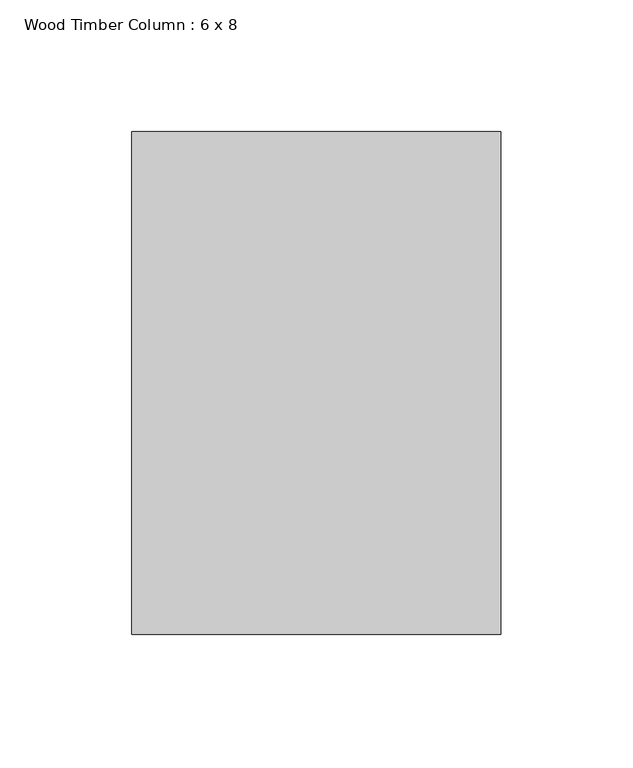
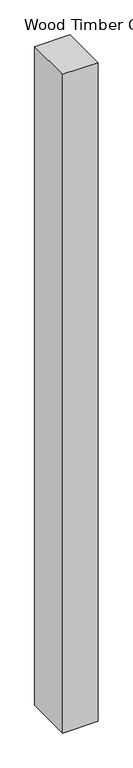
"""IFC4 building model written with IfcOpenShell, lengths in millimetres: column geometry, Wood Timber Column : 6 x 8."""

import ifcopenshell
import ifcopenshell.guid

model = None  # the IFC model being written
_history = None  # IfcOwnerHistory: only IFC2X3 demands one
_inside = {}  # id of a spatial element -> (the spatial element, [elements in it])
_under = {}  # id of a project, library or spatial element -> (it, [spatial elements below it])
_declared = {}  # id of a project -> (the project, [libraries it declares])
_typed = {}  # id of a type object -> (the type object, [elements of that type])
_made_of = {}  # id of a material, layer set ... -> (it, [elements and type objects made of it])


def new_model(schema):
    """Start an empty IFC model of exactly this schema.

    Asked for "IFC4X3", IfcOpenShell would pick the latest addendum, in which some entities
    have other attributes; the version numbers below select the first issue.
    IFC2X3 requires an IfcOwnerHistory on every rooted entity: one is made here for all.
    """
    global model, _history
    if schema == "IFC4X3":
        model = ifcopenshell.file(schema_version=(4, 3, 0, 0))
    else:
        model = ifcopenshell.file(schema=schema)
    _inside.clear()
    _under.clear()
    _declared.clear()
    _typed.clear()
    _made_of.clear()
    _history = None
    if model.schema == "IFC2X3":
        org = make("IfcOrganization", Name="unknown")
        user = make(
            "IfcPersonAndOrganization",
            ThePerson=make("IfcPerson", FamilyName="unknown"),
            TheOrganization=org,
        )
        app = make(
            "IfcApplication",
            ApplicationDeveloper=org,
            Version="unknown",
            ApplicationFullName="unknown",
            ApplicationIdentifier="unknown",
        )
        _history = make(
            "IfcOwnerHistory",
            OwningUser=user,
            OwningApplication=app,
            ChangeAction="ADDED",
            CreationDate=0,
        )
    return model


def make(cls, **values):
    """One entity of the class cls with the attributes given. An attribute that is None is left unset."""
    return model.create_entity(
        cls, **{name: value for name, value in values.items() if value is not None}
    )


def rooted(cls, **values):
    """An entity with a GlobalId (a new one), such as an element, a storey or a relation."""
    return make(cls, GlobalId=ifcopenshell.guid.new(), OwnerHistory=_history, **values)


def si_unit(unit_type, name, prefix=None):
    """IfcSIUnit, for example si_unit("LENGTHUNIT", "METRE", prefix="MILLI")."""
    return make("IfcSIUnit", UnitType=unit_type, Prefix=prefix, Name=name)


def assignment(units):
    """IfcUnitAssignment: the units of a project."""
    return None if units is None else make("IfcUnitAssignment", Units=units)


def point(xyz):
    """IfcCartesianPoint."""
    return None if xyz is None else make("IfcCartesianPoint", Coordinates=xyz)


def direction(xyz):
    """IfcDirection."""
    return None if xyz is None else make("IfcDirection", DirectionRatios=xyz)


def frame(location, z_axis=None, x_axis=None):
    """IfcAxis2Placement3D, a coordinate frame: its origin and axes. An axis left out is left unset."""
    return make(
        "IfcAxis2Placement3D",
        Location=point(location),
        Axis=direction(z_axis),
        RefDirection=direction(x_axis),
    )


def origin():
    """The frame at (0, 0, 0) with its axes left unset."""
    return frame((0.0, 0.0, 0.0))


def place(relative_to, where):
    """IfcLocalPlacement: puts the frame where relative to a parent placement (None: the world)."""
    return make(
        "IfcLocalPlacement", PlacementRelTo=relative_to, RelativePlacement=where
    )


def context(
    kind, dimensions, precision=None, world=None, true_north=None, identifier=None
):
    """IfcGeometricRepresentationContext, for example the 3D "Model" context."""
    return make(
        "IfcGeometricRepresentationContext",
        ContextIdentifier=identifier,
        ContextType=kind,
        CoordinateSpaceDimension=dimensions,
        Precision=precision,
        WorldCoordinateSystem=world,
        TrueNorth=true_north,
    )


def project(units=None, contexts=None):
    """IfcProject with its units and contexts."""
    return rooted(
        "IfcProject",
        Name="project",
        RepresentationContexts=contexts,
        UnitsInContext=assignment(units),
    )


def spatial(cls, under=None, at=None, **own):
    """A site, building, storey or space (cls), placed at a placement, below another one or the project."""
    s = rooted(cls, ObjectPlacement=at, **own)
    if under is not None:
        _under.setdefault(under.id(), (under, []))[1].append(s)
    return s


def polyline(points):
    """IfcPolyline through the points."""
    return make("IfcPolyline", Points=[point(p) for p in points])


def outline(outer, holes=None, kind="AREA"):
    """IfcArbitraryClosedProfileDef: a profile drawn as a closed curve; with holes, ...WithVoids."""
    if holes is None:
        return make("IfcArbitraryClosedProfileDef", ProfileType=kind, OuterCurve=outer)
    return make(
        "IfcArbitraryProfileDefWithVoids",
        ProfileType=kind,
        OuterCurve=outer,
        InnerCurves=holes,
    )


def extrude(swept, where, along, depth):
    """IfcExtrudedAreaSolid: the profile swept, set in the frame where, extruded along a direction by depth."""
    return make(
        "IfcExtrudedAreaSolid",
        SweptArea=swept,
        Position=where,
        ExtrudedDirection=direction(along),
        Depth=depth,
    )


def shape(context_of_items, identifier, shape_type, items):
    """IfcShapeRepresentation: the items that make up one representation, for example the "Body"."""
    return make(
        "IfcShapeRepresentation",
        ContextOfItems=context_of_items,
        RepresentationIdentifier=identifier,
        RepresentationType=shape_type,
        Items=items,
    )


def source(mapping_origin, context_of_items, identifier, shape_type, items):
    """IfcRepresentationMap: a shape defined once, which mapped items show again and again."""
    return make(
        "IfcRepresentationMap",
        MappingOrigin=mapping_origin,
        MappedRepresentation=shape(context_of_items, identifier, shape_type, items),
    )


def transform(
    local_origin,
    x_axis=None,
    y_axis=None,
    z_axis=None,
    scale=None,
    scale2=None,
    scale3=None,
    uniform=True,
):
    """IfcCartesianTransformationOperator3D, or its non-uniform kind. x_axis, y_axis, z_axis: its Axis1, 2, 3."""
    if uniform:
        return make(
            "IfcCartesianTransformationOperator3D",
            Axis1=direction(x_axis),
            Axis2=direction(y_axis),
            LocalOrigin=point(local_origin),
            Scale=scale,
            Axis3=direction(z_axis),
        )
    return make(
        "IfcCartesianTransformationOperator3DnonUniform",
        Axis1=direction(x_axis),
        Axis2=direction(y_axis),
        LocalOrigin=point(local_origin),
        Scale=scale,
        Axis3=direction(z_axis),
        Scale2=scale2,
        Scale3=scale3,
    )


def mapped(mapping_source, mapping_target):
    """IfcMappedItem: shows the shape of a source again, moved by a transform."""
    return make(
        "IfcMappedItem", MappingSource=mapping_source, MappingTarget=mapping_target
    )


def made_of(thing, what):
    """Note that an element or type object is made of a material, layer set ...; save() writes the relation."""
    if what is not None:
        _made_of.setdefault(what.id(), (what, []))[1].append(thing)
    return thing


def element(
    cls,
    number,
    at=None,
    inside=None,
    cuts=None,
    type_object=None,
    material=None,
    context=None,
    identifier="Body",
    shape_type=None,
    held_by="IfcProductDefinitionShape",
    body=None,
    shapes=None,
    **own,
):
    """One element of the class cls, such as IfcWall. Its Tag is "e" and its number.

    at: its placement. inside: the storey or other place that contains it. cuts: it is an
    opening in that element (IfcRelVoidsElement). A single representation is given by context,
    identifier, shape_type and body (its items); several are given by shapes. held_by: the class
    of the entity that holds the representations. save() writes the other relations.
    """
    e = rooted(cls, Tag="e%d" % number, ObjectPlacement=at, **own)
    if body is not None:
        shapes = [shape(context, identifier, shape_type, body)]
    if shapes is not None:
        e.Representation = make(held_by, Representations=shapes)
    if inside is not None:
        _inside.setdefault(inside.id(), (inside, []))[1].append(e)
    if cuts is not None:
        rooted(
            "IfcRelVoidsElement", RelatingBuildingElement=cuts, RelatedOpeningElement=e
        )
    if type_object is not None:
        _typed.setdefault(type_object.id(), (type_object, []))[1].append(e)
    return made_of(e, material)


def aggregate(whole, parts):
    """IfcRelAggregates: a whole, such as a stair, and the parts it consists of."""
    return rooted("IfcRelAggregates", RelatingObject=whole, RelatedObjects=parts)


def save(model, path):
    """Write the relations noted so far, then the file.

    IfcRelAggregates (storeys below a building ...), IfcRelContainedInSpatialStructure (elements
    in a storey), IfcRelDefinesByType, IfcRelAssociatesMaterial and IfcRelDeclares: one each for
    every whole, place, type object, material and project.
    """
    for whole, parts in _under.values():
        aggregate(whole, parts)
    for where, things in _inside.values():
        rooted(
            "IfcRelContainedInSpatialStructure",
            RelatedElements=things,
            RelatingStructure=where,
        )
    for kind, things in _typed.values():
        rooted("IfcRelDefinesByType", RelatedObjects=things, RelatingType=kind)
    for what, things in _made_of.values():
        rooted("IfcRelAssociatesMaterial", RelatedObjects=things, RelatingMaterial=what)
    for by, libraries in _declared.values():
        rooted("IfcRelDeclares", RelatingContext=by, RelatedDefinitions=libraries)
    model.write(path)


def wood_timber_column_6_x_8_dc19652e(model_context):
    return source(origin(), model_context, "Body", "SweptSolid", [
        extrude(outline(polyline([(69.85, -95.25), (-69.85, -95.25), (-69.85, 95.25), (69.85, 95.25), (69.85, -95.25)])), frame((0.0, 0.0, 2743.2), z_axis=(0.0, 0.0, 1.0), x_axis=(1.0, 0.0, 0.0)), (0.0, 0.0, 1.0), 2743.2),
    ])


if __name__ == "__main__":
    model = new_model("IFC4")
    model_context = context("Model", 3, world=origin())
    ifc_project = project(units=[si_unit("LENGTHUNIT", "METRE", prefix="MILLI")], contexts=[model_context])
    site = spatial("IfcSite", under=ifc_project)
    building = spatial("IfcBuilding", under=site)
    placement = place(None, origin())
    wood_timber_column_6_x_8_shape = wood_timber_column_6_x_8_dc19652e(model_context)
    element("IfcColumn", 1, ObjectType="Wood Timber Column : 6 x 8", at=placement, inside=building, context=model_context, shape_type="MappedRepresentation", body=[
        mapped(wood_timber_column_6_x_8_shape, transform((0.0, 0.0, 0.0), x_axis=(1.0, 0.0, 0.0), y_axis=(0.0, 1.0, 0.0), z_axis=(0.0, 0.0, 1.0))),
    ])
    save(model, "model.ifc")

# Revit data of these elements
# Type "Wood Timber Column : 6 x 8"
#   Assembly Code = "B1010200"
#   Depth = 0' - 7 1/2"
#   Width = 0' - 5 1/2"
#   Material = Softwood, Lumber (1)
# Element 1 (IfcColumn, "Wood Timber Column : 6 x 8")
#   Materials on its faces: "Softwood, Lumber (1)"
# Materials
#   "Softwood, Lumber (1)": class "Wood", colour RGB 234 198 147, transparency 0, Description = "Pinus Echinata", Cost = 0
